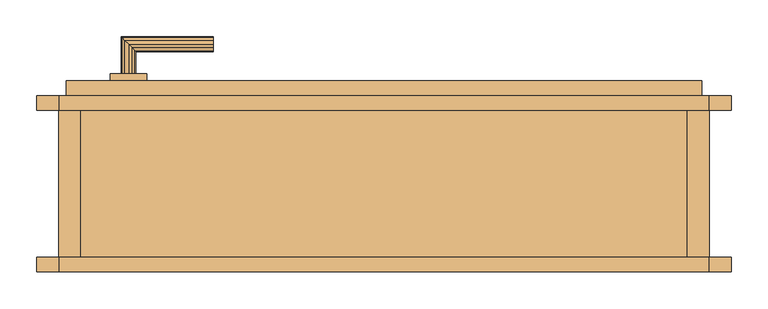
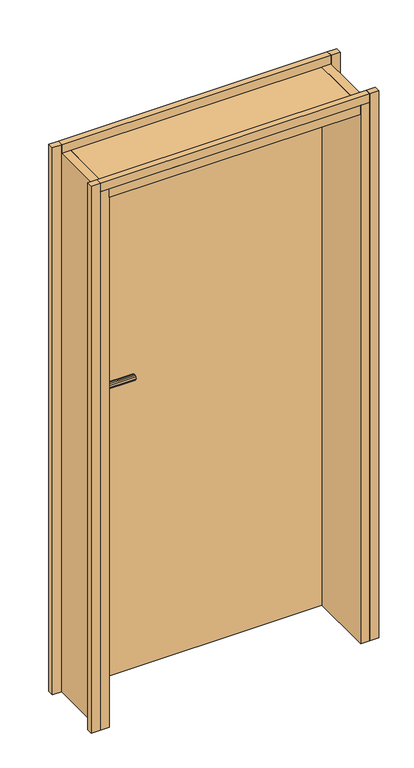
"""IFC4 building model written with IfcOpenShell, lengths in millimetres: door geometry, Tür."""

from ifc_helpers import new_model, si_unit, frame, origin, place, context, project, spatial, polyline, outline, extrude, faceted_brep, source, transform, mapped, element, save


def door_48d18684(model_context):
    return source(origin(), model_context, "Body", "SolidModel", [
        extrude(outline(polyline([(915.0, 220.0), (915.0, 200.0), (885.0, 200.0), (885.0, 220.0), (915.0, 220.0)])), frame((0.0, 0.0, 140.0), z_axis=(0.0, 0.0, 1.0), x_axis=(1.0, 0.0, 0.0)), (0.0, 0.0, 1.0), 1900.0),
        extrude(outline(polyline([(915.0, 0.0), (915.0, -20.0), (885.0, -20.0), (885.0, 0.0), (915.0, 0.0)])), frame((0.0, 0.0, 140.0), z_axis=(0.0, 0.0, 1.0), x_axis=(1.0, 0.0, 0.0)), (0.0, 0.0, 1.0), 1900.0),
        extrude(outline(polyline([(0.0, -20.0), (-30.0, -20.0), (-30.0, 0.0), (0.0, 0.0), (0.0, -20.0)])), frame((0.0, 0.0, 140.0), z_axis=(0.0, 0.0, 1.0), x_axis=(1.0, 0.0, 0.0)), (0.0, 0.0, 1.0), 1900.0),
        extrude(outline(polyline([(885.0, -20.0), (0.0, -20.0), (0.0, 0.0), (885.0, 0.0), (885.0, -20.0)])), frame((0.0, 0.0, 2010.0), z_axis=(0.0, 0.0, 1.0), x_axis=(1.0, 0.0, 0.0)), (0.0, 0.0, 1.0), 30.0),
        extrude(outline(polyline([(70.0, 190.0), (70.0, 200.0), (120.0, 200.0), (120.0, 190.0), (70.0, 190.0)])), frame((0.0, 0.0, 1050.0), z_axis=(0.0, 0.0, 1.0), x_axis=(1.0, 0.0, 0.0)), (0.0, 0.0, 1.0), 215.0),
        extrude(outline(polyline([(875.0, 200.0), (10.0, 200.0), (10.0, 240.0), (875.0, 240.0), (875.0, 200.0)])), frame((0.0, 0.0, 140.0), z_axis=(0.0, 0.0, 1.0), x_axis=(1.0, 0.0, 0.0)), (0.0, 0.0, 1.0), 1860.0),
        extrude(outline(polyline([(0.0, 200.0), (-30.0, 200.0), (-30.0, 220.0), (0.0, 220.0), (0.0, 200.0)])), frame((0.0, 0.0, 140.0), z_axis=(0.0, 0.0, 1.0), x_axis=(1.0, 0.0, 0.0)), (0.0, 0.0, 1.0), 1900.0),
        extrude(outline(polyline([(885.0, -20.0), (855.0, -20.0), (855.0, 220.0), (885.0, 220.0), (885.0, -20.0)])), frame((0.0, 0.0, 140.0), z_axis=(0.0, 0.0, 1.0), x_axis=(1.0, 0.0, 0.0)), (0.0, 0.0, 1.0), 1870.0),
        extrude(outline(polyline([(885.0, 200.0), (0.0, 200.0), (0.0, 220.0), (885.0, 220.0), (885.0, 200.0)])), frame((0.0, 0.0, 2010.0), z_axis=(0.0, 0.0, 1.0), x_axis=(1.0, 0.0, 0.0)), (0.0, 0.0, 1.0), 30.0),
        faceted_brep([(100.0, 250.0, 1198.660254), (95.0, 250.0, 1200.0), (90.0, 250.0, 1198.660254), (86.339746, 250.0, 1195.0), (85.0, 250.0, 1190.0), (86.339746, 250.0, 1185.0), (90.0, 250.0, 1181.339746), (95.0, 250.0, 1180.0), (100.0, 250.0, 1181.339746), (103.660254, 250.0, 1185.0), (105.0, 250.0, 1190.0), (103.660254, 250.0, 1195.0), (95.0, 290.0, 1200.0), (90.0, 295.0, 1198.660254), (86.339746, 298.660254, 1195.0), (85.0, 300.0, 1190.0), (86.339746, 298.660254, 1185.0), (90.0, 295.0, 1181.339746), (95.0, 290.0, 1180.0), (100.0, 285.0, 1181.339746), (103.660254, 281.339746, 1185.0), (105.0, 280.0, 1190.0), (103.660254, 281.339746, 1195.0), (100.0, 285.0, 1198.660254), (210.0, 295.0, 1198.660254), (210.0, 290.0, 1200.0), (210.0, 285.0, 1198.660254), (210.0, 281.339746, 1195.0), (210.0, 280.0, 1190.0), (210.0, 281.339746, 1185.0), (210.0, 285.0, 1181.339746), (210.0, 290.0, 1180.0), (210.0, 295.0, 1181.339746), (210.0, 298.660254, 1185.0), (210.0, 300.0, 1190.0), (210.0, 298.660254, 1195.0)], [[[0, 1, 2, 3, 4, 5, 6, 7, 8, 9, 10, 11]], [[2, 1, 12, 13]], [[3, 2, 13, 14]], [[4, 3, 14, 15]], [[5, 4, 15, 16]], [[6, 5, 16, 17]], [[7, 6, 17, 18]], [[8, 7, 18, 19]], [[9, 8, 19, 20]], [[10, 9, 20, 21]], [[11, 10, 21, 22]], [[0, 11, 22, 23]], [[1, 0, 23, 12]], [[24, 25, 26, 27, 28, 29, 30, 31, 32, 33, 34, 35]], [[13, 12, 25, 24]], [[14, 13, 24, 35]], [[15, 14, 35, 34]], [[16, 15, 34, 33]], [[17, 16, 33, 32]], [[18, 17, 32, 31]], [[19, 18, 31, 30]], [[20, 19, 30, 29]], [[21, 20, 29, 28]], [[22, 21, 28, 27]], [[23, 22, 27, 26]], [[12, 23, 26, 25]]]),
        extrude(outline(polyline([(855.0, -20.0), (30.0, -20.0), (30.0, 220.0), (855.0, 220.0), (855.0, -20.0)])), frame((0.0, 0.0, 1980.0), z_axis=(0.0, 0.0, 1.0), x_axis=(1.0, 0.0, 0.0)), (0.0, 0.0, 1.0), 30.0),
        extrude(outline(polyline([(30.0, -20.0), (0.0, -20.0), (0.0, 220.0), (30.0, 220.0), (30.0, -20.0)])), frame((0.0, 0.0, 140.0), z_axis=(0.0, 0.0, 1.0), x_axis=(1.0, 0.0, 0.0)), (0.0, 0.0, 1.0), 1870.0),
        extrude(outline(polyline([(120.0, 240.0), (70.0, 240.0), (70.0, 250.0), (120.0, 250.0), (120.0, 240.0)])), frame((0.0, 0.0, 1050.0), z_axis=(0.0, 0.0, 1.0), x_axis=(1.0, 0.0, 0.0)), (0.0, 0.0, 1.0), 215.0),
        faceted_brep([(90.0, 190.0, 1198.660254), (95.0, 190.0, 1200.0), (100.0, 190.0, 1198.660254), (103.660254, 190.0, 1195.0), (105.0, 190.0, 1190.0), (103.660254, 190.0, 1185.0), (100.0, 190.0, 1181.339746), (95.0, 190.0, 1180.0), (90.0, 190.0, 1181.339746), (86.339746, 190.0, 1185.0), (85.0, 190.0, 1190.0), (86.339746, 190.0, 1195.0), (95.0, 150.0, 1200.0), (90.0, 145.0, 1198.660254), (86.339746, 141.339746, 1195.0), (85.0, 140.0, 1190.0), (86.339746, 141.339746, 1185.0), (90.0, 145.0, 1181.339746), (95.0, 150.0, 1180.0), (100.0, 155.0, 1181.339746), (103.660254, 158.660254, 1185.0), (105.0, 160.0, 1190.0), (103.660254, 158.660254, 1195.0), (100.0, 155.0, 1198.660254), (210.0, 155.0, 1198.660254), (210.0, 150.0, 1200.0), (210.0, 145.0, 1198.660254), (210.0, 141.339746, 1195.0), (210.0, 140.0, 1190.0), (210.0, 141.339746, 1185.0), (210.0, 145.0, 1181.339746), (210.0, 150.0, 1180.0), (210.0, 155.0, 1181.339746), (210.0, 158.660254, 1185.0), (210.0, 160.0, 1190.0), (210.0, 158.660254, 1195.0)], [[[0, 1, 2, 3, 4, 5, 6, 7, 8, 9, 10, 11]], [[12, 1, 0, 13]], [[13, 0, 11, 14]], [[14, 11, 10, 15]], [[15, 10, 9, 16]], [[16, 9, 8, 17]], [[17, 8, 7, 18]], [[18, 7, 6, 19]], [[19, 6, 5, 20]], [[20, 5, 4, 21]], [[21, 4, 3, 22]], [[22, 3, 2, 23]], [[23, 2, 1, 12]], [[24, 25, 26, 27, 28, 29, 30, 31, 32, 33, 34, 35]], [[25, 12, 13, 26]], [[26, 13, 14, 27]], [[27, 14, 15, 28]], [[28, 15, 16, 29]], [[29, 16, 17, 30]], [[30, 17, 18, 31]], [[31, 18, 19, 32]], [[32, 19, 20, 33]], [[33, 20, 21, 34]], [[34, 21, 22, 35]], [[35, 22, 23, 24]], [[24, 23, 12, 25]]]),
    ])


if __name__ == "__main__":
    model = new_model("IFC4")
    model_context = context("Model", 3, world=origin())
    ifc_project = project(units=[si_unit("LENGTHUNIT", "METRE", prefix="MILLI")], contexts=[model_context])
    site = spatial("IfcSite", under=ifc_project)
    building = spatial("IfcBuilding", under=site)
    placement = place(None, origin())
    door_shape = door_48d18684(model_context)
    element("IfcDoor", 1, ObjectType="Tür", at=placement, inside=building, context=model_context, shape_type="MappedRepresentation", body=[
        mapped(door_shape, transform((0.0, 0.0, 0.0), x_axis=(1.0, 0.0, 0.0), y_axis=(0.0, 1.0, 0.0), z_axis=(0.0, 0.0, 1.0))),
    ])
    save(model, "model.ifc")

# Revit data of these elements
# Type "Tür"
#   Type Mark = "29"
# Element 1 (IfcDoor, "Tür")
#   Materials on its faces: "tuer_beschlag", "tuer_holzzarge"
# Materials
#   "tuer_beschlag": class "Unassigned", colour RGB 128 128 128, transparency 0
#   "tuer_holzzarge": class "Unassigned", colour RGB 255 255 255, transparency 0
